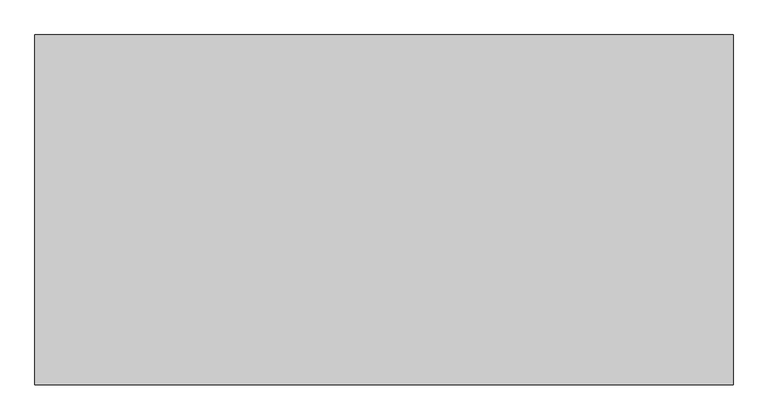
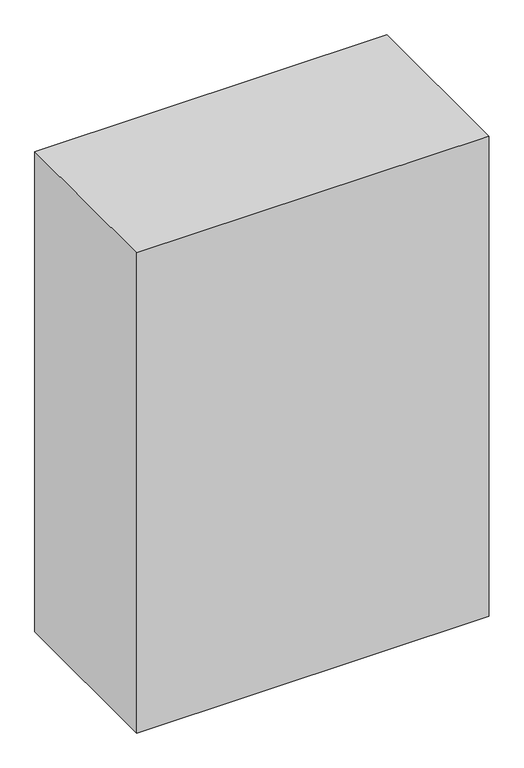
"""IFC4 building model written with IfcOpenShell, lengths in millimetres: proxy geometry, 0_3d."""

from ifc_helpers import new_model, si_unit, origin, origin_with_axes, place, context, project, spatial, polyline, outline, extrude, source, transform, mapped, element, save


def generic_models_c1c10271(model_context):
    return source(origin(), model_context, "Body", "SweptSolid", [
        extrude(outline(polyline([(1999.6864914, 0.0), (0.0, 0.0), (0.0, 1001.7), (1999.6864914, 1001.7), (1999.6864914, 0.0)])), origin_with_axes(), (0.0, 0.0, 1.0), 2880.0),
    ])


if __name__ == "__main__":
    model = new_model("IFC4")
    model_context = context("Model", 3, world=origin())
    ifc_project = project(units=[si_unit("LENGTHUNIT", "METRE", prefix="MILLI")], contexts=[model_context])
    site = spatial("IfcSite", under=ifc_project)
    building = spatial("IfcBuilding", under=site)
    placement = place(None, origin())
    generic_models_shape = generic_models_c1c10271(model_context)
    element("IfcBuildingElementProxy", 1, Name="0_3d", ObjectType="0_3d", at=placement, inside=building, context=model_context, shape_type="MappedRepresentation", body=[
        mapped(generic_models_shape, transform((0.0, 0.0, 0.0), x_axis=(1.0, 0.0, 0.0), y_axis=(0.0, 1.0, 0.0), z_axis=(0.0, 0.0, 1.0))),
    ])
    save(model, "model.ifc")

# Revit data of these elements
# Element 1 (IfcBuildingElementProxy, "0_3d")
#   Materials on its faces: "*1"
# Materials
#   "*1": class "Unassigned", colour RGB 175 175 175, transparency 0
